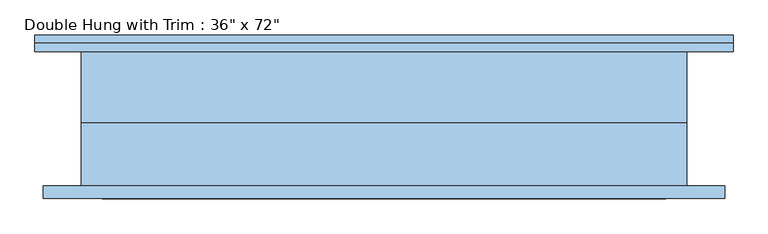
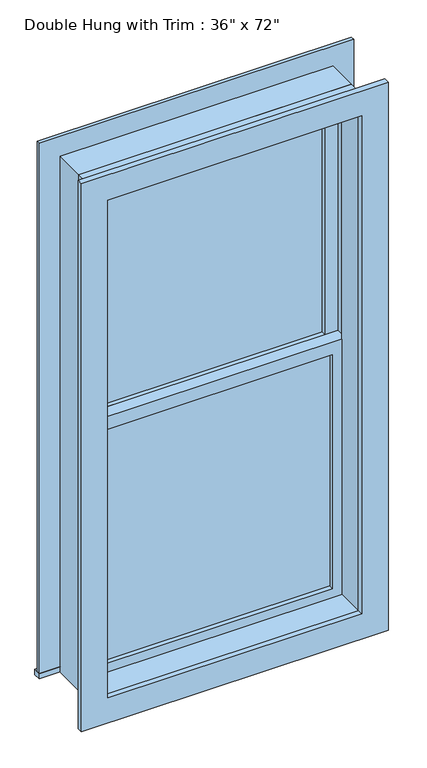
"""IFC4 building model written with IfcOpenShell, lengths in millimetres: window geometry."""

import ifcopenshell
import ifcopenshell.guid

model = None  # the IFC model being written
_history = None  # IfcOwnerHistory: only IFC2X3 demands one
_inside = {}  # id of a spatial element -> (the spatial element, [elements in it])
_under = {}  # id of a project, library or spatial element -> (it, [spatial elements below it])
_declared = {}  # id of a project -> (the project, [libraries it declares])
_typed = {}  # id of a type object -> (the type object, [elements of that type])
_made_of = {}  # id of a material, layer set ... -> (it, [elements and type objects made of it])


def new_model(schema):
    """Start an empty IFC model of exactly this schema.

    Asked for "IFC4X3", IfcOpenShell would pick the latest addendum, in which some entities
    have other attributes; the version numbers below select the first issue.
    IFC2X3 requires an IfcOwnerHistory on every rooted entity: one is made here for all.
    """
    global model, _history
    if schema == "IFC4X3":
        model = ifcopenshell.file(schema_version=(4, 3, 0, 0))
    else:
        model = ifcopenshell.file(schema=schema)
    _inside.clear()
    _under.clear()
    _declared.clear()
    _typed.clear()
    _made_of.clear()
    _history = None
    if model.schema == "IFC2X3":
        org = make("IfcOrganization", Name="unknown")
        user = make(
            "IfcPersonAndOrganization",
            ThePerson=make("IfcPerson", FamilyName="unknown"),
            TheOrganization=org,
        )
        app = make(
            "IfcApplication",
            ApplicationDeveloper=org,
            Version="unknown",
            ApplicationFullName="unknown",
            ApplicationIdentifier="unknown",
        )
        _history = make(
            "IfcOwnerHistory",
            OwningUser=user,
            OwningApplication=app,
            ChangeAction="ADDED",
            CreationDate=0,
        )
    return model


def make(cls, **values):
    """One entity of the class cls with the attributes given. An attribute that is None is left unset."""
    return model.create_entity(
        cls, **{name: value for name, value in values.items() if value is not None}
    )


def rooted(cls, **values):
    """An entity with a GlobalId (a new one), such as an element, a storey or a relation."""
    return make(cls, GlobalId=ifcopenshell.guid.new(), OwnerHistory=_history, **values)


def si_unit(unit_type, name, prefix=None):
    """IfcSIUnit, for example si_unit("LENGTHUNIT", "METRE", prefix="MILLI")."""
    return make("IfcSIUnit", UnitType=unit_type, Prefix=prefix, Name=name)


def assignment(units):
    """IfcUnitAssignment: the units of a project."""
    return None if units is None else make("IfcUnitAssignment", Units=units)


def point(xyz):
    """IfcCartesianPoint."""
    return None if xyz is None else make("IfcCartesianPoint", Coordinates=xyz)


def direction(xyz):
    """IfcDirection."""
    return None if xyz is None else make("IfcDirection", DirectionRatios=xyz)


def frame(location, z_axis=None, x_axis=None):
    """IfcAxis2Placement3D, a coordinate frame: its origin and axes. An axis left out is left unset."""
    return make(
        "IfcAxis2Placement3D",
        Location=point(location),
        Axis=direction(z_axis),
        RefDirection=direction(x_axis),
    )


def origin():
    """The frame at (0, 0, 0) with its axes left unset."""
    return frame((0.0, 0.0, 0.0))


def place(relative_to, where):
    """IfcLocalPlacement: puts the frame where relative to a parent placement (None: the world)."""
    return make(
        "IfcLocalPlacement", PlacementRelTo=relative_to, RelativePlacement=where
    )


def context(
    kind, dimensions, precision=None, world=None, true_north=None, identifier=None
):
    """IfcGeometricRepresentationContext, for example the 3D "Model" context."""
    return make(
        "IfcGeometricRepresentationContext",
        ContextIdentifier=identifier,
        ContextType=kind,
        CoordinateSpaceDimension=dimensions,
        Precision=precision,
        WorldCoordinateSystem=world,
        TrueNorth=true_north,
    )


def project(units=None, contexts=None):
    """IfcProject with its units and contexts."""
    return rooted(
        "IfcProject",
        Name="project",
        RepresentationContexts=contexts,
        UnitsInContext=assignment(units),
    )


def spatial(cls, under=None, at=None, **own):
    """A site, building, storey or space (cls), placed at a placement, below another one or the project."""
    s = rooted(cls, ObjectPlacement=at, **own)
    if under is not None:
        _under.setdefault(under.id(), (under, []))[1].append(s)
    return s


def polyline(points):
    """IfcPolyline through the points."""
    return make("IfcPolyline", Points=[point(p) for p in points])


def outline(outer, holes=None, kind="AREA"):
    """IfcArbitraryClosedProfileDef: a profile drawn as a closed curve; with holes, ...WithVoids."""
    if holes is None:
        return make("IfcArbitraryClosedProfileDef", ProfileType=kind, OuterCurve=outer)
    return make(
        "IfcArbitraryProfileDefWithVoids",
        ProfileType=kind,
        OuterCurve=outer,
        InnerCurves=holes,
    )


def extrude(swept, where, along, depth):
    """IfcExtrudedAreaSolid: the profile swept, set in the frame where, extruded along a direction by depth."""
    return make(
        "IfcExtrudedAreaSolid",
        SweptArea=swept,
        Position=where,
        ExtrudedDirection=direction(along),
        Depth=depth,
    )


def shape(context_of_items, identifier, shape_type, items):
    """IfcShapeRepresentation: the items that make up one representation, for example the "Body"."""
    return make(
        "IfcShapeRepresentation",
        ContextOfItems=context_of_items,
        RepresentationIdentifier=identifier,
        RepresentationType=shape_type,
        Items=items,
    )


def source(mapping_origin, context_of_items, identifier, shape_type, items):
    """IfcRepresentationMap: a shape defined once, which mapped items show again and again."""
    return make(
        "IfcRepresentationMap",
        MappingOrigin=mapping_origin,
        MappedRepresentation=shape(context_of_items, identifier, shape_type, items),
    )


def transform(
    local_origin,
    x_axis=None,
    y_axis=None,
    z_axis=None,
    scale=None,
    scale2=None,
    scale3=None,
    uniform=True,
):
    """IfcCartesianTransformationOperator3D, or its non-uniform kind. x_axis, y_axis, z_axis: its Axis1, 2, 3."""
    if uniform:
        return make(
            "IfcCartesianTransformationOperator3D",
            Axis1=direction(x_axis),
            Axis2=direction(y_axis),
            LocalOrigin=point(local_origin),
            Scale=scale,
            Axis3=direction(z_axis),
        )
    return make(
        "IfcCartesianTransformationOperator3DnonUniform",
        Axis1=direction(x_axis),
        Axis2=direction(y_axis),
        LocalOrigin=point(local_origin),
        Scale=scale,
        Axis3=direction(z_axis),
        Scale2=scale2,
        Scale3=scale3,
    )


def mapped(mapping_source, mapping_target):
    """IfcMappedItem: shows the shape of a source again, moved by a transform."""
    return make(
        "IfcMappedItem", MappingSource=mapping_source, MappingTarget=mapping_target
    )


def made_of(thing, what):
    """Note that an element or type object is made of a material, layer set ...; save() writes the relation."""
    if what is not None:
        _made_of.setdefault(what.id(), (what, []))[1].append(thing)
    return thing


def element(
    cls,
    number,
    at=None,
    inside=None,
    cuts=None,
    type_object=None,
    material=None,
    context=None,
    identifier="Body",
    shape_type=None,
    held_by="IfcProductDefinitionShape",
    body=None,
    shapes=None,
    **own,
):
    """One element of the class cls, such as IfcWall. Its Tag is "e" and its number.

    at: its placement. inside: the storey or other place that contains it. cuts: it is an
    opening in that element (IfcRelVoidsElement). A single representation is given by context,
    identifier, shape_type and body (its items); several are given by shapes. held_by: the class
    of the entity that holds the representations. save() writes the other relations.
    """
    e = rooted(cls, Tag="e%d" % number, ObjectPlacement=at, **own)
    if body is not None:
        shapes = [shape(context, identifier, shape_type, body)]
    if shapes is not None:
        e.Representation = make(held_by, Representations=shapes)
    if inside is not None:
        _inside.setdefault(inside.id(), (inside, []))[1].append(e)
    if cuts is not None:
        rooted(
            "IfcRelVoidsElement", RelatingBuildingElement=cuts, RelatedOpeningElement=e
        )
    if type_object is not None:
        _typed.setdefault(type_object.id(), (type_object, []))[1].append(e)
    return made_of(e, material)


def aggregate(whole, parts):
    """IfcRelAggregates: a whole, such as a stair, and the parts it consists of."""
    return rooted("IfcRelAggregates", RelatingObject=whole, RelatedObjects=parts)


def save(model, path):
    """Write the relations noted so far, then the file.

    IfcRelAggregates (storeys below a building ...), IfcRelContainedInSpatialStructure (elements
    in a storey), IfcRelDefinesByType, IfcRelAssociatesMaterial and IfcRelDeclares: one each for
    every whole, place, type object, material and project.
    """
    for whole, parts in _under.values():
        aggregate(whole, parts)
    for where, things in _inside.values():
        rooted(
            "IfcRelContainedInSpatialStructure",
            RelatedElements=things,
            RelatingStructure=where,
        )
    for kind, things in _typed.values():
        rooted("IfcRelDefinesByType", RelatedObjects=things, RelatingType=kind)
    for what, things in _made_of.values():
        rooted("IfcRelAssociatesMaterial", RelatedObjects=things, RelatingMaterial=what)
    for by, libraries in _declared.values():
        rooted("IfcRelDeclares", RelatingContext=by, RelatedDefinitions=libraries)
    model.write(path)


def window_d3583dd1(model_context):
    return source(origin(), model_context, "Body", "SweptSolid", [
        extrude(outline(polyline([(-393.7, 22.225), (393.7, 22.225), (393.7, 9.525), (-393.7, 9.525), (-393.7, 22.225)])), frame((0.0, 0.0, 368.3), z_axis=(0.0, 0.0, 1.0), x_axis=(1.0, 0.0, 0.0)), (0.0, 0.0, 1.0), 828.675),
        extrude(outline(polyline([(1241.425, -438.15), (323.85, -438.15), (323.85, 438.15), (1241.425, 438.15), (1241.425, -438.15)]), holes=[polyline([(1196.975, -393.7), (1196.975, 393.7), (368.3, 393.7), (368.3, -393.7), (1196.975, -393.7)])]), frame((0.0, -6.35, 0.0), z_axis=(0.0, 1.0, 0.0), x_axis=(0.0, 0.0, 1.0)), (0.0, 0.0, 1.0), 44.45),
        extrude(outline(polyline([(-527.05, 127.0), (527.05, 127.0), (527.05, 101.6), (-527.05, 101.6), (-527.05, 127.0)])), frame((0.0, 0.0, 304.8), z_axis=(0.0, 0.0, 1.0), x_axis=(1.0, 0.0, 0.0)), (0.0, 0.0, 1.0), 19.05),
        extrude(outline(polyline([(2114.55, -438.15), (2114.55, 438.15), (323.85, 438.15), (323.85, 527.05), (2203.45, 527.05), (2203.45, -527.05), (323.85, -527.05), (323.85, -438.15), (2114.55, -438.15)])), frame((0.0, 101.6, 0.0), z_axis=(0.0, 1.0, 0.0), x_axis=(0.0, 0.0, 1.0)), (0.0, 0.0, 1.0), 12.7),
        extrude(outline(polyline([(2190.75, 514.35), (2190.75, -514.35), (247.65, -514.35), (247.65, 514.35), (2190.75, 514.35)]), holes=[polyline([(2101.85, 425.45), (336.55, 425.45), (336.55, -425.45), (2101.85, -425.45), (2101.85, 425.45)])]), frame((0.0, -120.65, 0.0), z_axis=(0.0, 1.0, 0.0), x_axis=(0.0, 0.0, 1.0)), (0.0, 0.0, 1.0), 19.05),
        extrude(outline(polyline([(393.7, 53.975), (-393.7, 53.975), (-393.7, 66.675), (393.7, 66.675), (393.7, 53.975)])), frame((0.0, 0.0, 1241.425), z_axis=(0.0, 0.0, 1.0), x_axis=(1.0, 0.0, 0.0)), (0.0, 0.0, 1.0), 828.675),
        extrude(outline(polyline([(2114.55, -438.15), (1196.975, -438.15), (1196.975, 438.15), (2114.55, 438.15), (2114.55, -438.15)]), holes=[polyline([(2070.1, -393.7), (2070.1, 393.7), (1241.425, 393.7), (1241.425, -393.7), (2070.1, -393.7)])]), frame((0.0, 38.1, 0.0), z_axis=(0.0, 1.0, 0.0), x_axis=(0.0, 0.0, 1.0)), (0.0, 0.0, 1.0), 44.45),
        extrude(outline(polyline([(2133.6, -457.2), (304.8, -457.2), (304.8, 457.2), (2133.6, 457.2), (2133.6, -457.2)]), holes=[polyline([(2101.85, -425.45), (2101.85, 425.45), (336.55, 425.45), (336.55, -425.45), (2101.85, -425.45)])]), frame((0.0, -101.6, 0.0), z_axis=(0.0, 1.0, 0.0), x_axis=(0.0, 0.0, 1.0)), (0.0, 0.0, 1.0), 95.25),
        extrude(outline(polyline([(2133.6, 457.2), (2133.6, -457.2), (304.8, -457.2), (304.8, 457.2), (2133.6, 457.2)]), holes=[polyline([(2114.55, 438.15), (323.85, 438.15), (323.85, -438.15), (2114.55, -438.15), (2114.55, 438.15)])]), frame((0.0, -6.35, 0.0), z_axis=(0.0, 1.0, 0.0), x_axis=(0.0, 0.0, 1.0)), (0.0, 0.0, 1.0), 107.95),
    ])


if __name__ == "__main__":
    model = new_model("IFC4")
    model_context = context("Model", 3, world=origin())
    ifc_project = project(units=[si_unit("LENGTHUNIT", "METRE", prefix="MILLI")], contexts=[model_context])
    site = spatial("IfcSite", under=ifc_project)
    building = spatial("IfcBuilding", under=site)
    placement = place(None, origin())
    window_shape = window_d3583dd1(model_context)
    element("IfcWindow", 1, ObjectType="Double Hung with Trim : 36\" x 72\"", at=placement, inside=building, context=model_context, shape_type="MappedRepresentation", body=[
        mapped(window_shape, transform((0.0, 0.0, 0.0), x_axis=(1.0, 0.0, 0.0), y_axis=(0.0, 1.0, 0.0), z_axis=(0.0, 0.0, 1.0))),
    ])
    save(model, "model.ifc")

# Revit data of these elements
# Type "Double Hung with Trim : 36\" x 72\""
#   Type Mark = "21"
#   Construction Type Id = "GSP4R"
#   Assembly Code = "B2020100"
#   Analytic Construction = "1/8 in Pilkington single glazing"
#   Visual Light Transmittance = 0.9
#   Solar Heat Gain Coefficient = 0.78
#   Heat Transfer Coefficient (U) = 3.6886 W/(m²·K)
#   Height = 6' - 0"
#   Default Sill Height = 1' - 0"
#   Trim Projection - Ext. = 0' - 0 1/2"
#   Trim Projection - Int. = 0' - 0 3/4"
#   Trim Width - Exterior = 0' - 3 1/2"
#   Trim Width - Interior = 0' - 3 1/2"
#   Width = 3' - 0"
#   Window Inset = 0' - 0 3/4"
#   Glass Pane Material = Glass
#   Sash Material = Sash
#   Trim Exterior Material = Trim
#   Trim Interior Material = Trim
#   Wall Closure = (empty or 0)
# Element 1 (IfcWindow, "Double Hung with Trim : 36\" x 72\"")
#   Materials on its faces: "Sash", "Trim", "Glass"
# Materials
#   "Glass": class "Glass", colour RGB 0 128 192, transparency 0.75, Description = "Soda Lime Glass", Cost = 0
#   "Sash": class "Wood", colour RGB 224 178 126, transparency 0, Cost = 0
#   "Trim": class "Wood", colour RGB 224 178 126, transparency 0
